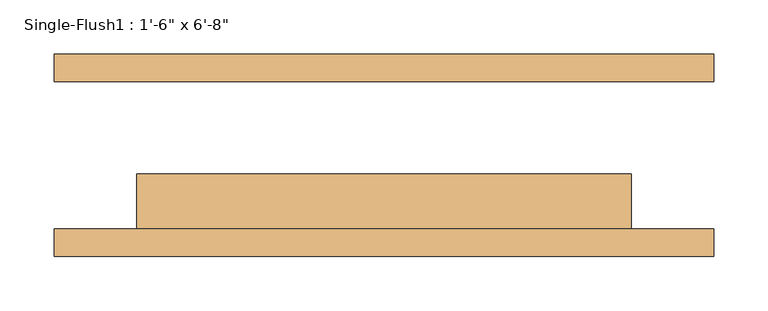
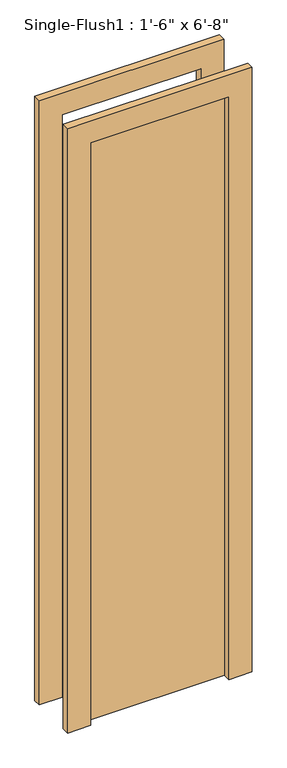
"""IFC4 building model written with IfcOpenShell, lengths in millimetres: door geometry."""

from ifc_helpers import new_model, si_unit, frame, origin, origin_with_axes, place, context, project, spatial, polyline, outline, extrude, source, transform, mapped, element, save


def door_7cdc0a33(model_context):
    return source(origin(), model_context, "Body", "SweptSolid", [
        extrude(outline(polyline([(2108.2, -304.8), (0.0, -304.8), (0.0, -228.6), (2032.0, -228.6), (2032.0, 228.6), (0.0, 228.6), (0.0, 304.8), (2108.2, 304.8), (2108.2, -304.8)])), frame((0.0, -93.6625, 0.0), z_axis=(0.0, 1.0, 0.0), x_axis=(0.0, 0.0, 1.0)), (0.0, 0.0, 1.0), 25.4),
        extrude(outline(polyline([(2108.2, 304.8), (2108.2, -304.8), (0.0, -304.8), (0.0, -228.6), (2032.0, -228.6), (2032.0, 228.6), (0.0, 228.6), (0.0, 304.8), (2108.2, 304.8)])), frame((0.0, 68.2625, 0.0), z_axis=(0.0, 1.0, 0.0), x_axis=(0.0, 0.0, 1.0)), (0.0, 0.0, 1.0), 25.4),
        extrude(outline(polyline([(228.6, -17.4625), (228.6, -68.2625), (-228.6, -68.2625), (-228.6, -17.4625), (228.6, -17.4625)])), origin_with_axes(), (0.0, 0.0, 1.0), 2032.0),
    ])


if __name__ == "__main__":
    model = new_model("IFC4")
    model_context = context("Model", 3, world=origin())
    ifc_project = project(units=[si_unit("LENGTHUNIT", "METRE", prefix="MILLI")], contexts=[model_context])
    site = spatial("IfcSite", under=ifc_project)
    building = spatial("IfcBuilding", under=site)
    placement = place(None, origin())
    door_shape = door_7cdc0a33(model_context)
    element("IfcDoor", 1, ObjectType="Single-Flush1 : 1'-6\" x 6'-8\"", at=placement, inside=building, context=model_context, shape_type="MappedRepresentation", body=[
        mapped(door_shape, transform((0.0, 0.0, 0.0), x_axis=(1.0, 0.0, 0.0), y_axis=(0.0, 1.0, 0.0), z_axis=(0.0, 0.0, 1.0))),
    ])
    save(model, "model.ifc")

# Revit data of these elements
# Type "Single-Flush1 : 1'-6\" x 6'-8\""
#   Type Mark = "D5"
#   Construction Type Id = "MDOOR"
#   Assembly Code = "C1020"
#   Analytic Construction = "Metal"
#   Thickness = 0' - 2"
#   Heat Transfer Coefficient (U) = 3.7021 W/(m²·K)
#   Height = 6' - 8"
#   Trim Projection Ext = 0' - 1"
#   Trim Projection Int = 0' - 1"
#   Trim Width = 0' - 3"
#   Width = 1' - 6"
#   Door Material = Door - Panel
#   Frame Material = Door - Frame
#   Visual Light Transmittance = 0
#   Solar Heat Gain Coefficient = 0
#   Function = (empty or 0)
#   Wall Closure = (empty or 0)
# Element 1 (IfcDoor, "Single-Flush1 : 1'-6\" x 6'-8\"")
#   Materials on its faces: "Door - Frame", "Door - Panel"
# Materials
#   "Door - Panel": class "Wood", colour RGB 210 159 95, transparency 0, Cost = 0
#   "Door - Frame": class "Miscellaneous", colour RGB 118 70 51, transparency 0, Cost = 0
